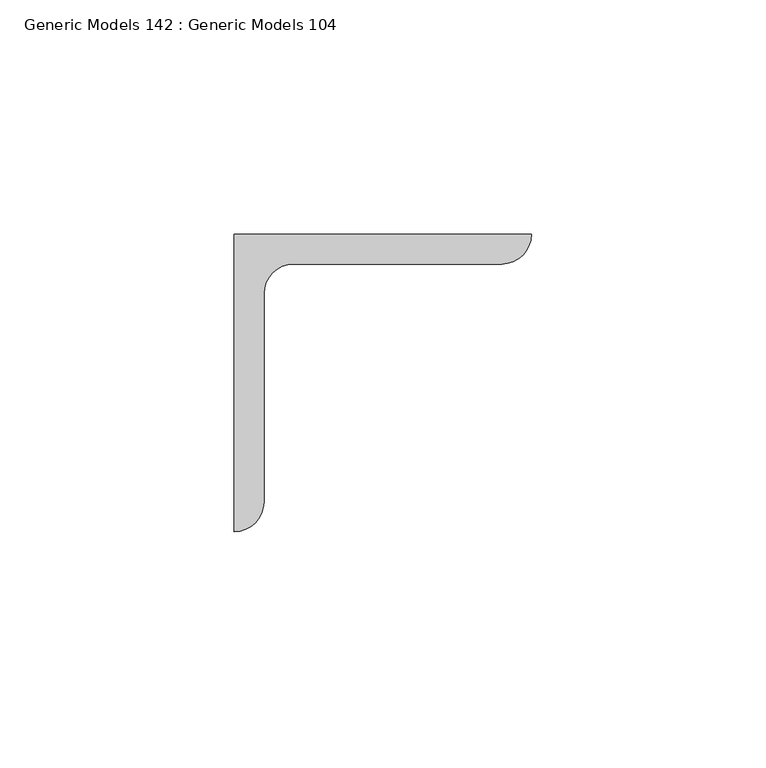
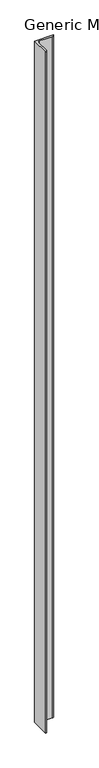
"""IFC4 building model written with IfcOpenShell, lengths in millimetres: proxy geometry, Generic Models 142 : Generic Models 104."""

import ifcopenshell
import ifcopenshell.guid

model = None  # the IFC model being written
_history = None  # IfcOwnerHistory: only IFC2X3 demands one
_inside = {}  # id of a spatial element -> (the spatial element, [elements in it])
_under = {}  # id of a project, library or spatial element -> (it, [spatial elements below it])
_declared = {}  # id of a project -> (the project, [libraries it declares])
_typed = {}  # id of a type object -> (the type object, [elements of that type])
_made_of = {}  # id of a material, layer set ... -> (it, [elements and type objects made of it])


def new_model(schema):
    """Start an empty IFC model of exactly this schema.

    Asked for "IFC4X3", IfcOpenShell would pick the latest addendum, in which some entities
    have other attributes; the version numbers below select the first issue.
    IFC2X3 requires an IfcOwnerHistory on every rooted entity: one is made here for all.
    """
    global model, _history
    if schema == "IFC4X3":
        model = ifcopenshell.file(schema_version=(4, 3, 0, 0))
    else:
        model = ifcopenshell.file(schema=schema)
    _inside.clear()
    _under.clear()
    _declared.clear()
    _typed.clear()
    _made_of.clear()
    _history = None
    if model.schema == "IFC2X3":
        org = make("IfcOrganization", Name="unknown")
        user = make(
            "IfcPersonAndOrganization",
            ThePerson=make("IfcPerson", FamilyName="unknown"),
            TheOrganization=org,
        )
        app = make(
            "IfcApplication",
            ApplicationDeveloper=org,
            Version="unknown",
            ApplicationFullName="unknown",
            ApplicationIdentifier="unknown",
        )
        _history = make(
            "IfcOwnerHistory",
            OwningUser=user,
            OwningApplication=app,
            ChangeAction="ADDED",
            CreationDate=0,
        )
    return model


def make(cls, **values):
    """One entity of the class cls with the attributes given. An attribute that is None is left unset."""
    return model.create_entity(
        cls, **{name: value for name, value in values.items() if value is not None}
    )


def rooted(cls, **values):
    """An entity with a GlobalId (a new one), such as an element, a storey or a relation."""
    return make(cls, GlobalId=ifcopenshell.guid.new(), OwnerHistory=_history, **values)


def si_unit(unit_type, name, prefix=None):
    """IfcSIUnit, for example si_unit("LENGTHUNIT", "METRE", prefix="MILLI")."""
    return make("IfcSIUnit", UnitType=unit_type, Prefix=prefix, Name=name)


def assignment(units):
    """IfcUnitAssignment: the units of a project."""
    return None if units is None else make("IfcUnitAssignment", Units=units)


def point(xyz):
    """IfcCartesianPoint."""
    return None if xyz is None else make("IfcCartesianPoint", Coordinates=xyz)


def direction(xyz):
    """IfcDirection."""
    return None if xyz is None else make("IfcDirection", DirectionRatios=xyz)


def frame(location, z_axis=None, x_axis=None):
    """IfcAxis2Placement3D, a coordinate frame: its origin and axes. An axis left out is left unset."""
    return make(
        "IfcAxis2Placement3D",
        Location=point(location),
        Axis=direction(z_axis),
        RefDirection=direction(x_axis),
    )


def frame_2d(location, x_axis=None):
    """IfcAxis2Placement2D, a coordinate frame in the plane: its origin and x axis."""
    return make(
        "IfcAxis2Placement2D", Location=point(location), RefDirection=direction(x_axis)
    )


def origin():
    """The frame at (0, 0, 0) with its axes left unset."""
    return frame((0.0, 0.0, 0.0))


def place(relative_to, where):
    """IfcLocalPlacement: puts the frame where relative to a parent placement (None: the world)."""
    return make(
        "IfcLocalPlacement", PlacementRelTo=relative_to, RelativePlacement=where
    )


def context(
    kind, dimensions, precision=None, world=None, true_north=None, identifier=None
):
    """IfcGeometricRepresentationContext, for example the 3D "Model" context."""
    return make(
        "IfcGeometricRepresentationContext",
        ContextIdentifier=identifier,
        ContextType=kind,
        CoordinateSpaceDimension=dimensions,
        Precision=precision,
        WorldCoordinateSystem=world,
        TrueNorth=true_north,
    )


def project(units=None, contexts=None):
    """IfcProject with its units and contexts."""
    return rooted(
        "IfcProject",
        Name="project",
        RepresentationContexts=contexts,
        UnitsInContext=assignment(units),
    )


def spatial(cls, under=None, at=None, **own):
    """A site, building, storey or space (cls), placed at a placement, below another one or the project."""
    s = rooted(cls, ObjectPlacement=at, **own)
    if under is not None:
        _under.setdefault(under.id(), (under, []))[1].append(s)
    return s


def polyline(points):
    """IfcPolyline through the points."""
    return make("IfcPolyline", Points=[point(p) for p in points])


def circle_curve(where, radius):
    """IfcCircle in the frame where."""
    return make("IfcCircle", Position=where, Radius=radius)


def trimmed(basis, trim1, trim2, sense, master):
    """IfcTrimmedCurve: the piece of a basis curve between two trims."""
    return make(
        "IfcTrimmedCurve",
        BasisCurve=basis,
        Trim1=trim1,
        Trim2=trim2,
        SenseAgreement=sense,
        MasterRepresentation=master,
    )


def segment(curve, same_sense, transition):
    """IfcCompositeCurveSegment."""
    return make(
        "IfcCompositeCurveSegment",
        Transition=transition,
        SameSense=same_sense,
        ParentCurve=curve,
    )


def composite_curve(segments, self_intersect=None):
    """IfcCompositeCurve: segments joined end to end."""
    return make("IfcCompositeCurve", Segments=segments, SelfIntersect=self_intersect)


def outline(outer, holes=None, kind="AREA"):
    """IfcArbitraryClosedProfileDef: a profile drawn as a closed curve; with holes, ...WithVoids."""
    if holes is None:
        return make("IfcArbitraryClosedProfileDef", ProfileType=kind, OuterCurve=outer)
    return make(
        "IfcArbitraryProfileDefWithVoids",
        ProfileType=kind,
        OuterCurve=outer,
        InnerCurves=holes,
    )


def extrude(swept, where, along, depth):
    """IfcExtrudedAreaSolid: the profile swept, set in the frame where, extruded along a direction by depth."""
    return make(
        "IfcExtrudedAreaSolid",
        SweptArea=swept,
        Position=where,
        ExtrudedDirection=direction(along),
        Depth=depth,
    )


def shape(context_of_items, identifier, shape_type, items):
    """IfcShapeRepresentation: the items that make up one representation, for example the "Body"."""
    return make(
        "IfcShapeRepresentation",
        ContextOfItems=context_of_items,
        RepresentationIdentifier=identifier,
        RepresentationType=shape_type,
        Items=items,
    )


def source(mapping_origin, context_of_items, identifier, shape_type, items):
    """IfcRepresentationMap: a shape defined once, which mapped items show again and again."""
    return make(
        "IfcRepresentationMap",
        MappingOrigin=mapping_origin,
        MappedRepresentation=shape(context_of_items, identifier, shape_type, items),
    )


def transform(
    local_origin,
    x_axis=None,
    y_axis=None,
    z_axis=None,
    scale=None,
    scale2=None,
    scale3=None,
    uniform=True,
):
    """IfcCartesianTransformationOperator3D, or its non-uniform kind. x_axis, y_axis, z_axis: its Axis1, 2, 3."""
    if uniform:
        return make(
            "IfcCartesianTransformationOperator3D",
            Axis1=direction(x_axis),
            Axis2=direction(y_axis),
            LocalOrigin=point(local_origin),
            Scale=scale,
            Axis3=direction(z_axis),
        )
    return make(
        "IfcCartesianTransformationOperator3DnonUniform",
        Axis1=direction(x_axis),
        Axis2=direction(y_axis),
        LocalOrigin=point(local_origin),
        Scale=scale,
        Axis3=direction(z_axis),
        Scale2=scale2,
        Scale3=scale3,
    )


def mapped(mapping_source, mapping_target):
    """IfcMappedItem: shows the shape of a source again, moved by a transform."""
    return make(
        "IfcMappedItem", MappingSource=mapping_source, MappingTarget=mapping_target
    )


def made_of(thing, what):
    """Note that an element or type object is made of a material, layer set ...; save() writes the relation."""
    if what is not None:
        _made_of.setdefault(what.id(), (what, []))[1].append(thing)
    return thing


def element(
    cls,
    number,
    at=None,
    inside=None,
    cuts=None,
    type_object=None,
    material=None,
    context=None,
    identifier="Body",
    shape_type=None,
    held_by="IfcProductDefinitionShape",
    body=None,
    shapes=None,
    **own,
):
    """One element of the class cls, such as IfcWall. Its Tag is "e" and its number.

    at: its placement. inside: the storey or other place that contains it. cuts: it is an
    opening in that element (IfcRelVoidsElement). A single representation is given by context,
    identifier, shape_type and body (its items); several are given by shapes. held_by: the class
    of the entity that holds the representations. save() writes the other relations.
    """
    e = rooted(cls, Tag="e%d" % number, ObjectPlacement=at, **own)
    if body is not None:
        shapes = [shape(context, identifier, shape_type, body)]
    if shapes is not None:
        e.Representation = make(held_by, Representations=shapes)
    if inside is not None:
        _inside.setdefault(inside.id(), (inside, []))[1].append(e)
    if cuts is not None:
        rooted(
            "IfcRelVoidsElement", RelatingBuildingElement=cuts, RelatedOpeningElement=e
        )
    if type_object is not None:
        _typed.setdefault(type_object.id(), (type_object, []))[1].append(e)
    return made_of(e, material)


def aggregate(whole, parts):
    """IfcRelAggregates: a whole, such as a stair, and the parts it consists of."""
    return rooted("IfcRelAggregates", RelatingObject=whole, RelatedObjects=parts)


def save(model, path):
    """Write the relations noted so far, then the file.

    IfcRelAggregates (storeys below a building ...), IfcRelContainedInSpatialStructure (elements
    in a storey), IfcRelDefinesByType, IfcRelAssociatesMaterial and IfcRelDeclares: one each for
    every whole, place, type object, material and project.
    """
    for whole, parts in _under.values():
        aggregate(whole, parts)
    for where, things in _inside.values():
        rooted(
            "IfcRelContainedInSpatialStructure",
            RelatedElements=things,
            RelatingStructure=where,
        )
    for kind, things in _typed.values():
        rooted("IfcRelDefinesByType", RelatedObjects=things, RelatingType=kind)
    for what, things in _made_of.values():
        rooted("IfcRelAssociatesMaterial", RelatedObjects=things, RelatingMaterial=what)
    for by, libraries in _declared.values():
        rooted("IfcRelDeclares", RelatingContext=by, RelatedDefinitions=libraries)
    model.write(path)


def generic_models_142_generic_models_104_5ef028d8(model_context):
    return source(origin(), model_context, "Body", "SweptSolid", [
        extrude(outline(composite_curve([segment(polyline([(32326.8940778, 41071.1196612), (32390.3940778, 41071.1196612)]), True, "CONTINUOUS"), segment(trimmed(circle_curve(frame_2d((32384.0440778, 41071.1196612)), 6.35), [point((32390.3940778, 41071.1196612))], [point((32384.0440778, 41064.7696612))], False, "CARTESIAN"), True, "CONTINUOUS"), segment(polyline([(32384.0440778, 41064.7696612), (32339.5940778, 41064.7696612)]), True, "CONTINUOUS"), segment(trimmed(circle_curve(frame_2d((32339.5940778, 41058.4196612)), 6.35), [point((32339.5940778, 41064.7696612))], [point((32333.2440778, 41058.4196612))], True, "CARTESIAN"), True, "CONTINUOUS"), segment(polyline([(32333.2440778, 41058.4196612), (32333.2440778, 41013.9696612)]), True, "CONTINUOUS"), segment(trimmed(circle_curve(frame_2d((32326.8940778, 41013.9696612)), 6.35), [point((32333.2440778, 41013.9696612))], [point((32326.8940778, 41007.6196612))], False, "CARTESIAN"), True, "CONTINUOUS"), segment(polyline([(32326.8940778, 41007.6196612), (32326.8940778, 41071.1196612)]), True, "CONTINUOUS")], self_intersect=False)), frame((0.0, 0.0, 266407.9), z_axis=(0.0, 0.0, 1.0), x_axis=(1.0, 0.0, 0.0)), (0.0, 0.0, 1.0), 2432.1044757),
    ])


if __name__ == "__main__":
    model = new_model("IFC4")
    model_context = context("Model", 3, world=origin())
    ifc_project = project(units=[si_unit("LENGTHUNIT", "METRE", prefix="MILLI")], contexts=[model_context])
    site = spatial("IfcSite", under=ifc_project)
    building = spatial("IfcBuilding", under=site)
    placement = place(None, origin())
    generic_models_142_generic_models_104_shape = generic_models_142_generic_models_104_5ef028d8(model_context)
    element("IfcBuildingElementProxy", 1, Name="Generic Models 142 : Generic Models 104", ObjectType="Generic Models 142 : Generic Models 104", at=placement, inside=building, context=model_context, shape_type="MappedRepresentation", body=[
        mapped(generic_models_142_generic_models_104_shape, transform((0.0, 0.0, 0.0), x_axis=(1.0, 0.0, 0.0), y_axis=(0.0, 1.0, 0.0), z_axis=(0.0, 0.0, 1.0))),
    ])
    save(model, "model.ifc")

# Revit data of these elements
# Element 1 (IfcBuildingElementProxy, "Generic Models 142 : Generic Models 104")
#   Materials on its faces: "(2) BACK/BACK GALVANIZED ANGLES (2) L2 1/2 X 2 1/2 X 1/4\")"
# Materials
#   "(2) BACK/BACK GALVANIZED ANGLES (2) L2 1/2 X 2 1/2 X 1/4\")": class "Unassigned", colour RGB 211 211 211, transparency 0, Cost = 0
